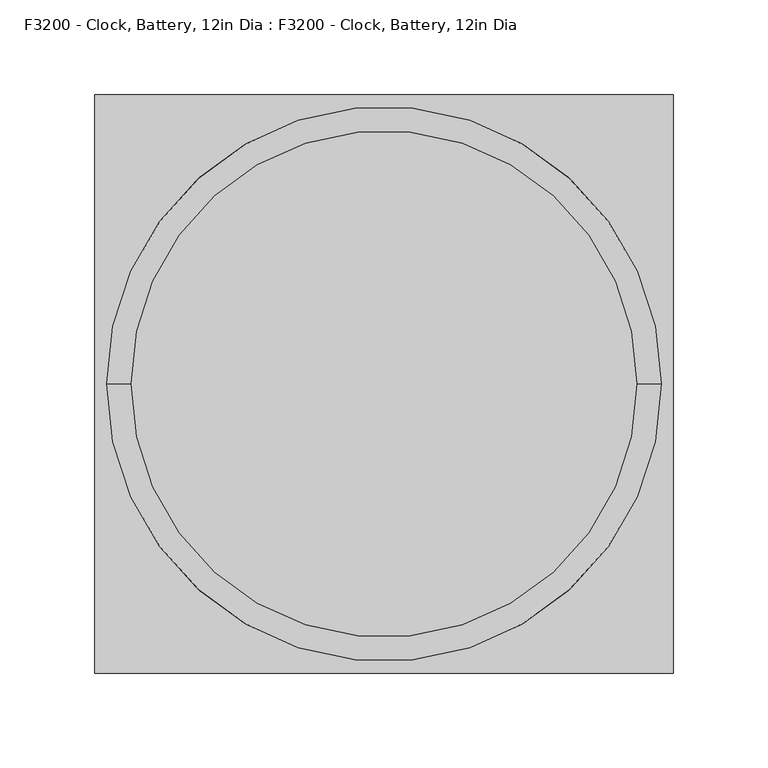
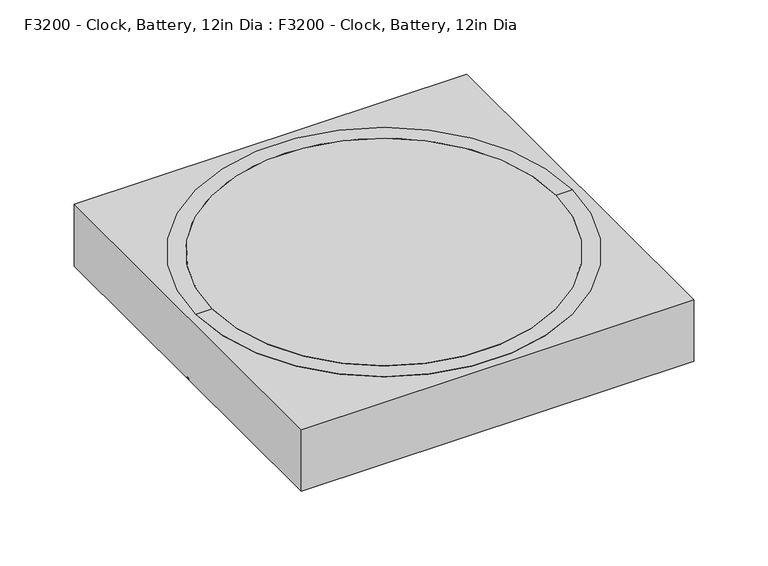
"""IFC4 building model written with IfcOpenShell, lengths in millimetres: proxy geometry, F3200 - Clock, Battery, 12in Dia : F3200 - Clock, Battery, 12in Dia."""

import ifcopenshell
import ifcopenshell.guid

model = None  # the IFC model being written
_history = None  # IfcOwnerHistory: only IFC2X3 demands one
_inside = {}  # id of a spatial element -> (the spatial element, [elements in it])
_under = {}  # id of a project, library or spatial element -> (it, [spatial elements below it])
_declared = {}  # id of a project -> (the project, [libraries it declares])
_typed = {}  # id of a type object -> (the type object, [elements of that type])
_made_of = {}  # id of a material, layer set ... -> (it, [elements and type objects made of it])


def new_model(schema):
    """Start an empty IFC model of exactly this schema.

    Asked for "IFC4X3", IfcOpenShell would pick the latest addendum, in which some entities
    have other attributes; the version numbers below select the first issue.
    IFC2X3 requires an IfcOwnerHistory on every rooted entity: one is made here for all.
    """
    global model, _history
    if schema == "IFC4X3":
        model = ifcopenshell.file(schema_version=(4, 3, 0, 0))
    else:
        model = ifcopenshell.file(schema=schema)
    _inside.clear()
    _under.clear()
    _declared.clear()
    _typed.clear()
    _made_of.clear()
    _history = None
    if model.schema == "IFC2X3":
        org = make("IfcOrganization", Name="unknown")
        user = make(
            "IfcPersonAndOrganization",
            ThePerson=make("IfcPerson", FamilyName="unknown"),
            TheOrganization=org,
        )
        app = make(
            "IfcApplication",
            ApplicationDeveloper=org,
            Version="unknown",
            ApplicationFullName="unknown",
            ApplicationIdentifier="unknown",
        )
        _history = make(
            "IfcOwnerHistory",
            OwningUser=user,
            OwningApplication=app,
            ChangeAction="ADDED",
            CreationDate=0,
        )
    return model


def make(cls, **values):
    """One entity of the class cls with the attributes given. An attribute that is None is left unset."""
    return model.create_entity(
        cls, **{name: value for name, value in values.items() if value is not None}
    )


def rooted(cls, **values):
    """An entity with a GlobalId (a new one), such as an element, a storey or a relation."""
    return make(cls, GlobalId=ifcopenshell.guid.new(), OwnerHistory=_history, **values)


def si_unit(unit_type, name, prefix=None):
    """IfcSIUnit, for example si_unit("LENGTHUNIT", "METRE", prefix="MILLI")."""
    return make("IfcSIUnit", UnitType=unit_type, Prefix=prefix, Name=name)


def assignment(units):
    """IfcUnitAssignment: the units of a project."""
    return None if units is None else make("IfcUnitAssignment", Units=units)


def point(xyz):
    """IfcCartesianPoint."""
    return None if xyz is None else make("IfcCartesianPoint", Coordinates=xyz)


def direction(xyz):
    """IfcDirection."""
    return None if xyz is None else make("IfcDirection", DirectionRatios=xyz)


def frame(location, z_axis=None, x_axis=None):
    """IfcAxis2Placement3D, a coordinate frame: its origin and axes. An axis left out is left unset."""
    return make(
        "IfcAxis2Placement3D",
        Location=point(location),
        Axis=direction(z_axis),
        RefDirection=direction(x_axis),
    )


def frame_2d(location, x_axis=None):
    """IfcAxis2Placement2D, a coordinate frame in the plane: its origin and x axis."""
    return make(
        "IfcAxis2Placement2D", Location=point(location), RefDirection=direction(x_axis)
    )


def origin():
    """The frame at (0, 0, 0) with its axes left unset."""
    return frame((0.0, 0.0, 0.0))


def origin_with_axes():
    """The frame at (0, 0, 0) with the z axis (0, 0, 1) and the x axis (1, 0, 0) written out."""
    return frame((0.0, 0.0, 0.0), z_axis=(0.0, 0.0, 1.0), x_axis=(1.0, 0.0, 0.0))


def place(relative_to, where):
    """IfcLocalPlacement: puts the frame where relative to a parent placement (None: the world)."""
    return make(
        "IfcLocalPlacement", PlacementRelTo=relative_to, RelativePlacement=where
    )


def context(
    kind, dimensions, precision=None, world=None, true_north=None, identifier=None
):
    """IfcGeometricRepresentationContext, for example the 3D "Model" context."""
    return make(
        "IfcGeometricRepresentationContext",
        ContextIdentifier=identifier,
        ContextType=kind,
        CoordinateSpaceDimension=dimensions,
        Precision=precision,
        WorldCoordinateSystem=world,
        TrueNorth=true_north,
    )


def project(units=None, contexts=None):
    """IfcProject with its units and contexts."""
    return rooted(
        "IfcProject",
        Name="project",
        RepresentationContexts=contexts,
        UnitsInContext=assignment(units),
    )


def spatial(cls, under=None, at=None, **own):
    """A site, building, storey or space (cls), placed at a placement, below another one or the project."""
    s = rooted(cls, ObjectPlacement=at, **own)
    if under is not None:
        _under.setdefault(under.id(), (under, []))[1].append(s)
    return s


def polyline(points):
    """IfcPolyline through the points."""
    return make("IfcPolyline", Points=[point(p) for p in points])


def circle_curve(where, radius):
    """IfcCircle in the frame where."""
    return make("IfcCircle", Position=where, Radius=radius)


def trimmed(basis, trim1, trim2, sense, master):
    """IfcTrimmedCurve: the piece of a basis curve between two trims."""
    return make(
        "IfcTrimmedCurve",
        BasisCurve=basis,
        Trim1=trim1,
        Trim2=trim2,
        SenseAgreement=sense,
        MasterRepresentation=master,
    )


def segment(curve, same_sense, transition):
    """IfcCompositeCurveSegment."""
    return make(
        "IfcCompositeCurveSegment",
        Transition=transition,
        SameSense=same_sense,
        ParentCurve=curve,
    )


def composite_curve(segments, self_intersect=None):
    """IfcCompositeCurve: segments joined end to end."""
    return make("IfcCompositeCurve", Segments=segments, SelfIntersect=self_intersect)


def outline(outer, holes=None, kind="AREA"):
    """IfcArbitraryClosedProfileDef: a profile drawn as a closed curve; with holes, ...WithVoids."""
    if holes is None:
        return make("IfcArbitraryClosedProfileDef", ProfileType=kind, OuterCurve=outer)
    return make(
        "IfcArbitraryProfileDefWithVoids",
        ProfileType=kind,
        OuterCurve=outer,
        InnerCurves=holes,
    )


def extrude(swept, where, along, depth):
    """IfcExtrudedAreaSolid: the profile swept, set in the frame where, extruded along a direction by depth."""
    return make(
        "IfcExtrudedAreaSolid",
        SweptArea=swept,
        Position=where,
        ExtrudedDirection=direction(along),
        Depth=depth,
    )


def shape(context_of_items, identifier, shape_type, items):
    """IfcShapeRepresentation: the items that make up one representation, for example the "Body"."""
    return make(
        "IfcShapeRepresentation",
        ContextOfItems=context_of_items,
        RepresentationIdentifier=identifier,
        RepresentationType=shape_type,
        Items=items,
    )


def source(mapping_origin, context_of_items, identifier, shape_type, items):
    """IfcRepresentationMap: a shape defined once, which mapped items show again and again."""
    return make(
        "IfcRepresentationMap",
        MappingOrigin=mapping_origin,
        MappedRepresentation=shape(context_of_items, identifier, shape_type, items),
    )


def transform(
    local_origin,
    x_axis=None,
    y_axis=None,
    z_axis=None,
    scale=None,
    scale2=None,
    scale3=None,
    uniform=True,
):
    """IfcCartesianTransformationOperator3D, or its non-uniform kind. x_axis, y_axis, z_axis: its Axis1, 2, 3."""
    if uniform:
        return make(
            "IfcCartesianTransformationOperator3D",
            Axis1=direction(x_axis),
            Axis2=direction(y_axis),
            LocalOrigin=point(local_origin),
            Scale=scale,
            Axis3=direction(z_axis),
        )
    return make(
        "IfcCartesianTransformationOperator3DnonUniform",
        Axis1=direction(x_axis),
        Axis2=direction(y_axis),
        LocalOrigin=point(local_origin),
        Scale=scale,
        Axis3=direction(z_axis),
        Scale2=scale2,
        Scale3=scale3,
    )


def mapped(mapping_source, mapping_target):
    """IfcMappedItem: shows the shape of a source again, moved by a transform."""
    return make(
        "IfcMappedItem", MappingSource=mapping_source, MappingTarget=mapping_target
    )


def made_of(thing, what):
    """Note that an element or type object is made of a material, layer set ...; save() writes the relation."""
    if what is not None:
        _made_of.setdefault(what.id(), (what, []))[1].append(thing)
    return thing


def element(
    cls,
    number,
    at=None,
    inside=None,
    cuts=None,
    type_object=None,
    material=None,
    context=None,
    identifier="Body",
    shape_type=None,
    held_by="IfcProductDefinitionShape",
    body=None,
    shapes=None,
    **own,
):
    """One element of the class cls, such as IfcWall. Its Tag is "e" and its number.

    at: its placement. inside: the storey or other place that contains it. cuts: it is an
    opening in that element (IfcRelVoidsElement). A single representation is given by context,
    identifier, shape_type and body (its items); several are given by shapes. held_by: the class
    of the entity that holds the representations. save() writes the other relations.
    """
    e = rooted(cls, Tag="e%d" % number, ObjectPlacement=at, **own)
    if body is not None:
        shapes = [shape(context, identifier, shape_type, body)]
    if shapes is not None:
        e.Representation = make(held_by, Representations=shapes)
    if inside is not None:
        _inside.setdefault(inside.id(), (inside, []))[1].append(e)
    if cuts is not None:
        rooted(
            "IfcRelVoidsElement", RelatingBuildingElement=cuts, RelatedOpeningElement=e
        )
    if type_object is not None:
        _typed.setdefault(type_object.id(), (type_object, []))[1].append(e)
    return made_of(e, material)


def aggregate(whole, parts):
    """IfcRelAggregates: a whole, such as a stair, and the parts it consists of."""
    return rooted("IfcRelAggregates", RelatingObject=whole, RelatedObjects=parts)


def save(model, path):
    """Write the relations noted so far, then the file.

    IfcRelAggregates (storeys below a building ...), IfcRelContainedInSpatialStructure (elements
    in a storey), IfcRelDefinesByType, IfcRelAssociatesMaterial and IfcRelDeclares: one each for
    every whole, place, type object, material and project.
    """
    for whole, parts in _under.values():
        aggregate(whole, parts)
    for where, things in _inside.values():
        rooted(
            "IfcRelContainedInSpatialStructure",
            RelatedElements=things,
            RelatingStructure=where,
        )
    for kind, things in _typed.values():
        rooted("IfcRelDefinesByType", RelatedObjects=things, RelatingType=kind)
    for what, things in _made_of.values():
        rooted("IfcRelAssociatesMaterial", RelatedObjects=things, RelatingMaterial=what)
    for by, libraries in _declared.values():
        rooted("IfcRelDeclares", RelatingContext=by, RelatedDefinitions=libraries)
    model.write(path)


def plane_surface(at):
    """IfcPlane: the flat surface through the origin of the frame at, square to its z axis."""
    return make("IfcPlane", Position=at)


def revolved_surface(curve, axis_point, axis_direction):
    """IfcSurfaceOfRevolution: the curve turned about the line through axis_point along axis_direction."""
    return make(
        "IfcSurfaceOfRevolution",
        SweptCurve=make("IfcArbitraryOpenProfileDef", ProfileType="CURVE", Curve=curve),
        AxisPosition=make("IfcAxis1Placement", Location=point(axis_point), Axis=direction(axis_direction)),
    )


def advanced_brep(points, edges, surfaces, faces):
    """IfcAdvancedBrep: a solid bounded by faces that lie on surfaces and meet in shared edges.

    An edge is (start, end): straight between two places in points (the first is 0);
    or (start, end, curve); or (start, end, curve, False) where it runs against its curve.
    A face is (place in surfaces, loops), or (place, loops, False) where it looks against
    its surface's normal. A loop lists edges by number (the first is 1), with a minus sign
    where the edge is run from its end to its start. The first loop is the outer one.
    """
    corners = [point(p) for p in points]
    vertices = [make("IfcVertexPoint", VertexGeometry=c) for c in corners]
    made = []
    for start, end, *more in edges:
        made.append(
            make(
                "IfcEdgeCurve",
                EdgeStart=vertices[start],
                EdgeEnd=vertices[end],
                EdgeGeometry=more[0] if more else make("IfcPolyline", Points=[corners[start], corners[end]]),
                SameSense=more[1] if len(more) > 1 else True,
            )
        )
    hull = []
    for where, loops, *sense in faces:
        bounds = []
        for j, loop in enumerate(loops):
            ring = [make("IfcOrientedEdge", EdgeElement=made[abs(k) - 1], Orientation=k > 0) for k in loop]
            bounds.append(
                make(
                    "IfcFaceOuterBound" if j == 0 else "IfcFaceBound",
                    Bound=make("IfcEdgeLoop", EdgeList=ring),
                    Orientation=True,
                )
            )
        hull.append(make("IfcAdvancedFace", Bounds=bounds, FaceSurface=surfaces[where], SameSense=sense[0] if sense else True))
    return make("IfcAdvancedBrep", Outer=make("IfcClosedShell", CfsFaces=hull))


def f3200_clock_battery_12in_dia_f3200_clock_battery_12in_dia_9ad0a7d1(model_context):
    return source(origin(), model_context, "Body", "SolidModel", [
        extrude(outline(composite_curve([segment(trimmed(circle_curve(frame_2d((0.0, -152.4)), 133.35), [point((-133.35, -152.4))], [point((133.35, -152.4))], False, "CARTESIAN"), True, "CONTINUOUS"), segment(trimmed(circle_curve(frame_2d((0.0, -152.4)), 133.35), [point((133.35, -152.4))], [point((-133.35, -152.4))], False, "CARTESIAN"), True, "CONTINUOUS")], self_intersect=False)), frame((0.0, 0.0, 44.45), z_axis=(0.0, 0.0, 1.0), x_axis=(1.0, 0.0, 0.0)), (0.0, 0.0, 1.0), 6.35),
        advanced_brep(
        [(0.0, -152.4, 0.0), (-152.4, -152.4, 0.0), (152.4, -152.4, 0.0), (-133.35, -152.4, 44.45), (0.0, -152.4, 44.45), (133.35, -152.4, 44.45), (-133.35, -152.4, 50.8), (133.35, -152.4, 50.8), (-146.05, -152.4, 50.8), (146.05, -152.4, 50.8)],
        [
            (0, 1),
            (1, 2, circle_curve(frame((0.0, -152.4, 0.0), z_axis=(0.0, 0.0, -1.0), x_axis=(1.0, 0.0, 0.0)), 152.4)),
            (2, 0),
            (2, 1, circle_curve(frame((0.0, -152.4, 0.0), z_axis=(0.0, 0.0, -1.0), x_axis=(1.0, 0.0, 0.0)), 152.4)),
            (3, 4),
            (4, 5),
            (5, 3, circle_curve(frame((0.0, -152.4, 44.45), z_axis=(0.0, 0.0, 1.0), x_axis=(1.0, 0.0, 0.0)), 133.35)),
            (3, 5, circle_curve(frame((0.0, -152.4, 44.45), z_axis=(0.0, 0.0, 1.0), x_axis=(1.0, 0.0, 0.0)), 133.35)),
            (6, 3),
            (5, 7),
            (7, 6, circle_curve(frame((0.0, -152.4, 50.8), z_axis=(0.0, 0.0, 1.0), x_axis=(1.0, 0.0, 0.0)), 133.35)),
            (6, 7, circle_curve(frame((0.0, -152.4, 50.8), z_axis=(0.0, 0.0, 1.0), x_axis=(1.0, 0.0, 0.0)), 133.35)),
            (8, 6),
            (7, 9),
            (9, 8, circle_curve(frame((0.0, -152.4, 50.8), z_axis=(0.0, 0.0, 1.0), x_axis=(1.0, 0.0, 0.0)), 146.05)),
            (8, 9, circle_curve(frame((0.0, -152.4, 50.8), z_axis=(0.0, 0.0, 1.0), x_axis=(1.0, 0.0, 0.0)), 146.05)),
            (1, 8),
            (9, 2),
        ],
        [
            plane_surface(frame((0.0, -152.4, 0.0), z_axis=(0.0, 0.0, -1.0), x_axis=(1.0, 0.0, 0.0))),
            plane_surface(frame((0.0, -152.4, 44.45), z_axis=(0.0, 0.0, 1.0), x_axis=(1.0, 0.0, 0.0))),
            revolved_surface(polyline([(133.35, -152.4, 44.45), (133.35, -152.4, 50.8)]), (0.0, -152.4, 0.0), (0.0, 0.0, -1.0)),
            plane_surface(frame((0.0, -152.4, 50.8), z_axis=(0.0, 0.0, 1.0), x_axis=(1.0, 0.0, 0.0))),
            revolved_surface(polyline([(146.05, -152.4, 50.8), (152.4, -152.4, 0.0)]), (0.0, -152.4, 0.0), (0.0, 0.0, -1.0)),
        ],
        [
            (0, [[1, 2, 3]]),
            (0, [[-3, 4, -1]]),
            (1, [[5, 6, 7]]),
            (1, [[-6, -5, 8]]),
            (2, [[9, -7, 10, 11]]),
            (2, [[-10, -8, -9, 12]]),
            (3, [[13, -11, 14, 15]]),
            (3, [[-14, -12, -13, 16]]),
            (4, [[17, -15, 18, -2]]),
            (4, [[-18, -16, -17, -4]]),
        ],
    ),
        extrude(outline(polyline([(152.4, -304.8), (-152.4, -304.8), (-152.4, 0.0), (152.4, 0.0), (152.4, -304.8)])), origin_with_axes(), (0.0, 0.0, 1.0), 50.8),
    ])


if __name__ == "__main__":
    model = new_model("IFC4")
    model_context = context("Model", 3, world=origin())
    ifc_project = project(units=[si_unit("LENGTHUNIT", "METRE", prefix="MILLI")], contexts=[model_context])
    site = spatial("IfcSite", under=ifc_project)
    building = spatial("IfcBuilding", under=site)
    placement = place(None, origin())
    f3200_clock_battery_12in_dia_f3200_clock_battery_12in_dia_shape = f3200_clock_battery_12in_dia_f3200_clock_battery_12in_dia_9ad0a7d1(model_context)
    element("IfcBuildingElementProxy", 1, Name="F3200 - Clock, Battery, 12in Dia : F3200 - Clock, Battery, 12in Dia", ObjectType="F3200 - Clock, Battery, 12in Dia : F3200 - Clock, Battery, 12in Dia", at=placement, inside=building, context=model_context, shape_type="MappedRepresentation", body=[
        mapped(f3200_clock_battery_12in_dia_f3200_clock_battery_12in_dia_shape, transform((0.0, 0.0, 0.0), x_axis=(1.0, 0.0, 0.0), y_axis=(0.0, 1.0, 0.0), z_axis=(0.0, 0.0, 1.0))),
    ])
    save(model, "model.ifc")

# Revit data of these elements
# Project information
#   Room Abbreviation = "DNTG1"
#   Room Description = "Dental Treatment Room, General (DNTG1)"
#   Sheets - Total = "5"
#   Project Issue Date = "Issue Date"
#   Project Status = "Project Status"
#   Client Name = "Owner"
#   Project Address = "Enter address here"
#   Project Name = "Project Name"
#   Project Number = "Project Number"
#   Publication Date = "30-Jan-15"
# Type "F3200 - Clock, Battery, 12in Dia : F3200 - Clock, Battery, 12in Dia"
#   Watts2 = "0"
#   Watts1 = "0"
#   Unit_Issue = "EA"
#   UTIL_6_Misc = "-"
#   UTIL_5_NonMedGas = "-"
#   UTIL_4_MiscGas = "-"
#   UTIL_3_MedGas = "-"
#   UTIL_2_Elec = "-"
#   UTIL_1_WaterDrain = "-"
#   Nomenclature = "Clock, Battery, 12\" Diameter"
#   NSN = "6645"
#   Location [instance default] = ""
#   JSN = "F3200"
#   Fund_Source_VA = "-"
#   Fund_Source_Navy = "-"
#   Fund_Source_Army = "-"
#   Fund_Source_AF = "-"
#   ELEC_Volts2 = "0"
#   ELEC_Volts1 = "0"
#   ELEC_Phase2 = "0"
#   ELEC_Phase1 = "0"
#   ELEC_HertzSwitch = "0"
#   ELEC_HertzDependent = "0"
#   ELEC_Hertz = "0"
#   ELEC_Amps2 = "0"
#   ELEC_Amps1 = "0"
#   DetailDescription = "Clock, 12\" diameter. Round surface, easy to read numbers with sweep second hand. Wall mounted unit for use when impractical to install a fully synchronized clock system. Battery operated, (batteries not included)."
#   CAT_VA = "C"
#   CAT_Navy = "C"
#   CAT_IHS = "-"
#   CAT_Army = "C"
#   CAT_AF = "C"
#   BTUperhour = "0"
#   radius = 0' - 6"
#   Weight_IP = 2
#   Default Elevation = 6' - 6"
#   DIM_Width_IP = 1' - 0"
#   DIM_Height_IP = 1' - 0"
#   DIM_Depth_IP = 0' - 2"
#   Assembly Code = ""
# Element 1 (IfcBuildingElementProxy, "F3200 - Clock, Battery, 12in Dia : F3200 - Clock, Battery, 12in Dia")
#   Location = "DNTG1"
#   Materials on its faces: "EquipSpace", "White"
# Materials
#   "EquipSpace": class "Unassigned", colour RGB 221 217 195, transparency 0.5
#   "White": class "Miscellaneous", colour RGB 255 255 255, transparency 0.4
